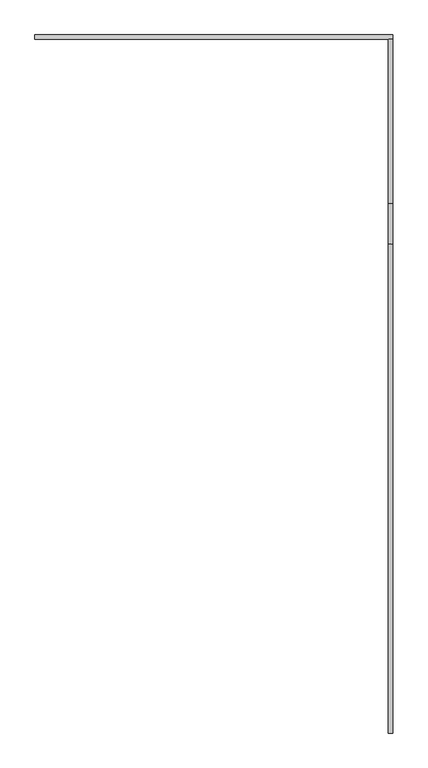
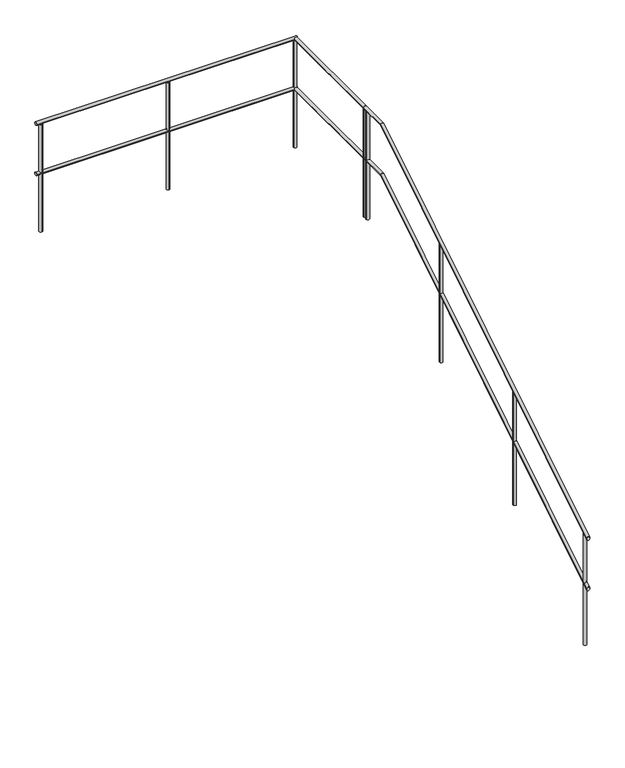
"""IFC4 building model written with IfcOpenShell, lengths in millimetres: railing geometry."""

from ifc_helpers import new_model, si_unit, point, frame, frame_2d, origin, place, context, project, spatial, circle_curve, ellipse_curve, trimmed, segment, composite_curve, outline, extrude, source, transform, mapped, element, save
from ifc_brep_helpers import plane_surface, cylinder_surface, advanced_brep


def railing_f57b0715(model_context):
    return source(origin(), model_context, "Body", "SolidModel", [
        advanced_brep(
        [(12685.1052251, 14699.5208589, 456.3396197), (12655.1052251, 14699.5208589, 456.3396197), (12685.1052251, 18339.5208589, 2547.0), (12655.1052251, 18339.5208589, 2547.0), (12685.1052251, 18063.8019306, 2547.0), (12655.1052251, 18063.8019306, 2547.0)],
        [
            (0, 1, ellipse_curve(frame((12670.1052251, 14699.5208589, 456.3396197), z_axis=(0.0, -1.0, 0.0), x_axis=(0.0, 0.0, -1.0)), 17.6603803, 15.0)),
            (1, 0, ellipse_curve(frame((12670.1052251, 14699.5208589, 456.3396197), z_axis=(0.0, -1.0, 0.0), x_axis=(0.0, 0.0, -1.0)), 17.6603803, 15.0)),
            (2, 3, circle_curve(frame((12670.1052251, 18339.5208589, 2547.0), z_axis=(0.0, 1.0, 0.0), x_axis=(-1.0, 0.0, 0.0)), 15.0)),
            (3, 2, circle_curve(frame((12670.1052251, 18339.5208589, 2547.0), z_axis=(0.0, 1.0, 0.0), x_axis=(-1.0, 0.0, 0.0)), 15.0)),
            (0, 4),
            (4, 5, ellipse_curve(frame((12670.1052251, 18063.8019306, 2547.0), z_axis=(0.0, -0.9616025257983003, -0.2744459552959912), x_axis=(0.0, 0.2744459552959914, -0.9616025257983002)), 15.5989607, 15.0)),
            (5, 1),
            (5, 4, ellipse_curve(frame((12670.1052251, 18063.8019306, 2547.0), z_axis=(0.0, -0.9616025257983003, -0.2744459552959912), x_axis=(0.0, 0.2744459552959914, -0.9616025257983002)), 15.5989607, 15.0)),
            (4, 2),
            (3, 5),
        ],
        [
            plane_surface(frame((12670.1052251, 14699.5208589, 474.0), z_axis=(0.0, -1.0, 0.0), x_axis=(0.0, 0.0, 1.0))),
            plane_surface(frame((12670.1052251, 18339.5208589, 2562.0), z_axis=(0.0, 1.0, 0.0), x_axis=(0.0, 0.0, 1.0))),
            cylinder_surface(frame((12670.1052251, 14707.4380966, 461.2596175), z_axis=(0.0, -0.8493588352433417, -0.5278158476155052), x_axis=(-1.0, 0.0, 0.0)), 15.0),
            cylinder_surface(frame((12670.1052251, 18059.5208589, 2547.0), z_axis=(0.0, -1.0, 0.0), x_axis=(-1.0, 0.0, 0.0)), 15.0),
        ],
        [
            (0, [[1, 2]]),
            (1, [[3, 4]]),
            (2, [[-1, 5, 6, 7]]),
            (2, [[-2, -7, 8, -5]]),
            (3, [[-6, 9, -4, 10]]),
            (3, [[-8, -10, -3, -9]]),
        ],
    ),
        advanced_brep(
        [(12685.1052251, 18339.5208589, 2547.0), (12655.1052251, 18339.5208589, 2547.0), (12685.1052251, 19469.5208589, 2547.0), (12655.1052251, 19469.5208589, 2547.0)],
        [
            (0, 1, circle_curve(frame((12670.1052251, 18339.5208589, 2547.0), z_axis=(0.0, -1.0, 0.0), x_axis=(-1.0, 0.0, 0.0)), 15.0)),
            (1, 0, circle_curve(frame((12670.1052251, 18339.5208589, 2547.0), z_axis=(0.0, -1.0, 0.0), x_axis=(-1.0, 0.0, 0.0)), 15.0)),
            (2, 3, circle_curve(frame((12670.1052251, 19469.5208589, 2547.0), z_axis=(0.0, 1.0, 0.0), x_axis=(-1.0, 0.0, 0.0)), 15.0)),
            (3, 2, circle_curve(frame((12670.1052251, 19469.5208589, 2547.0), z_axis=(0.0, 1.0, 0.0), x_axis=(-1.0, 0.0, 0.0)), 15.0)),
            (0, 2),
            (3, 1),
        ],
        [
            plane_surface(frame((12670.1052251, 18339.5208589, 2562.0), z_axis=(0.0, -1.0, 0.0), x_axis=(0.0, 0.0, 1.0))),
            plane_surface(frame((12670.1052251, 19469.5208589, 2562.0), z_axis=(0.0, 1.0, 0.0), x_axis=(0.0, 0.0, 1.0))),
            cylinder_surface(frame((12670.1052251, 18339.5208589, 2547.0), z_axis=(0.0, -1.0, 0.0), x_axis=(-1.0, 0.0, 0.0)), 15.0),
        ],
        [
            (0, [[1, 2]]),
            (1, [[3, 4]]),
            (2, [[-1, 5, -4, 6]]),
            (2, [[-2, -6, -3, -5]]),
        ],
    ),
        advanced_brep(
        [(12685.1052251, 19499.5208589, 2547.0), (12685.1052251, 19469.5208589, 2547.0), (10225.1052251, 19499.5208589, 2547.0), (10225.1052251, 19469.5208589, 2547.0)],
        [
            (0, 1, circle_curve(frame((12685.1052251, 19484.5208589, 2547.0), z_axis=(1.0, 0.0, 0.0), x_axis=(0.0, -1.0, 0.0)), 15.0)),
            (1, 0, circle_curve(frame((12685.1052251, 19484.5208589, 2547.0), z_axis=(1.0, 0.0, 0.0), x_axis=(0.0, -1.0, 0.0)), 15.0)),
            (2, 3, circle_curve(frame((10225.1052251, 19484.5208589, 2547.0), z_axis=(-1.0, 0.0, 0.0), x_axis=(0.0, -1.0, 0.0)), 15.0)),
            (3, 2, circle_curve(frame((10225.1052251, 19484.5208589, 2547.0), z_axis=(-1.0, 0.0, 0.0), x_axis=(0.0, -1.0, 0.0)), 15.0)),
            (0, 2),
            (3, 1),
        ],
        [
            plane_surface(frame((12685.1052251, 19484.5208589, 2562.0), z_axis=(1.0, 0.0, 0.0), x_axis=(0.0, -1.0, 0.0))),
            plane_surface(frame((10225.1052251, 19484.5208589, 2562.0), z_axis=(-1.0, 0.0, 0.0), x_axis=(0.0, -1.0, 0.0))),
            cylinder_surface(frame((12685.1052251, 19484.5208589, 2547.0), z_axis=(1.0, 0.0, 0.0), x_axis=(0.0, -1.0, 0.0)), 15.0),
        ],
        [
            (0, [[1, 2]]),
            (1, [[3, 4]]),
            (2, [[-1, 5, -4, 6]]),
            (2, [[-2, -6, -3, -5]]),
        ],
    ),
        advanced_brep(
        [(12685.1052251, 14699.5208589, 956.3396197), (12655.1052251, 14699.5208589, 956.3396197), (12685.1052251, 18063.8019306, 3047.0), (12655.1052251, 18063.8019306, 3047.0), (12685.1052251, 18339.5208589, 3047.0), (12655.1052251, 18339.5208589, 3047.0)],
        [
            (0, 1, ellipse_curve(frame((12670.1052251, 14699.5208589, 956.3396197), z_axis=(0.0, -1.0, 0.0), x_axis=(0.0, 0.0, -1.0)), 17.6603803, 15.0)),
            (1, 0, ellipse_curve(frame((12670.1052251, 14699.5208589, 956.3396197), z_axis=(0.0, -1.0, 0.0), x_axis=(0.0, 0.0, -1.0)), 17.6603803, 15.0)),
            (0, 2),
            (2, 3, ellipse_curve(frame((12670.1052251, 18063.8019306, 3047.0), z_axis=(0.0, -0.9616025257983003, -0.2744459552959912), x_axis=(0.0, 0.2744459552959914, -0.9616025257983002)), 15.5989607, 15.0)),
            (3, 1),
            (3, 2, ellipse_curve(frame((12670.1052251, 18063.8019306, 3047.0), z_axis=(0.0, -0.9616025257983003, -0.2744459552959912), x_axis=(0.0, 0.2744459552959914, -0.9616025257983002)), 15.5989607, 15.0)),
            (4, 5, circle_curve(frame((12670.1052251, 18339.5208589, 3047.0), z_axis=(0.0, 1.0, 0.0), x_axis=(-1.0, 0.0, 0.0)), 15.0)),
            (5, 4, circle_curve(frame((12670.1052251, 18339.5208589, 3047.0), z_axis=(0.0, 1.0, 0.0), x_axis=(-1.0, 0.0, 0.0)), 15.0)),
            (2, 4),
            (5, 3),
        ],
        [
            plane_surface(frame((12670.1052251, 14699.5208589, 974.0), z_axis=(0.0, -1.0, 0.0), x_axis=(0.0, 0.0, 1.0))),
            cylinder_surface(frame((12670.1052251, 14707.4380966, 961.2596175), z_axis=(0.0, -0.8493588352433417, -0.5278158476155052), x_axis=(-1.0, 0.0, 0.0)), 15.0),
            plane_surface(frame((12670.1052251, 18339.5208589, 3062.0), z_axis=(0.0, 1.0, 0.0), x_axis=(0.0, 0.0, 1.0))),
            cylinder_surface(frame((12670.1052251, 18059.5208589, 3047.0), z_axis=(0.0, -1.0, 0.0), x_axis=(-1.0, 0.0, 0.0)), 15.0),
        ],
        [
            (0, [[1, 2]]),
            (1, [[-1, 3, 4, 5]]),
            (1, [[-2, -5, 6, -3]]),
            (2, [[7, 8]]),
            (3, [[-4, 9, -8, 10]]),
            (3, [[-6, -10, -7, -9]]),
        ],
    ),
        advanced_brep(
        [(12685.1052251, 18339.5208589, 3047.0), (12655.1052251, 18339.5208589, 3047.0), (12685.1052251, 19469.5208589, 3047.0), (12655.1052251, 19469.5208589, 3047.0)],
        [
            (0, 1, circle_curve(frame((12670.1052251, 18339.5208589, 3047.0), z_axis=(0.0, -1.0, 0.0), x_axis=(-1.0, 0.0, 0.0)), 15.0)),
            (1, 0, circle_curve(frame((12670.1052251, 18339.5208589, 3047.0), z_axis=(0.0, -1.0, 0.0), x_axis=(-1.0, 0.0, 0.0)), 15.0)),
            (2, 3, circle_curve(frame((12670.1052251, 19469.5208589, 3047.0), z_axis=(0.0, 1.0, 0.0), x_axis=(-1.0, 0.0, 0.0)), 15.0)),
            (3, 2, circle_curve(frame((12670.1052251, 19469.5208589, 3047.0), z_axis=(0.0, 1.0, 0.0), x_axis=(-1.0, 0.0, 0.0)), 15.0)),
            (0, 2),
            (3, 1),
        ],
        [
            plane_surface(frame((12670.1052251, 18339.5208589, 3062.0), z_axis=(0.0, -1.0, 0.0), x_axis=(0.0, 0.0, 1.0))),
            plane_surface(frame((12670.1052251, 19469.5208589, 3062.0), z_axis=(0.0, 1.0, 0.0), x_axis=(0.0, 0.0, 1.0))),
            cylinder_surface(frame((12670.1052251, 18339.5208589, 3047.0), z_axis=(0.0, -1.0, 0.0), x_axis=(-1.0, 0.0, 0.0)), 15.0),
        ],
        [
            (0, [[1, 2]]),
            (1, [[3, 4]]),
            (2, [[-1, 5, -4, 6]]),
            (2, [[-2, -6, -3, -5]]),
        ],
    ),
        advanced_brep(
        [(12685.1052251, 19499.5208589, 3047.0), (12685.1052251, 19469.5208589, 3047.0), (10225.1052251, 19499.5208589, 3047.0), (10225.1052251, 19469.5208589, 3047.0)],
        [
            (0, 1, circle_curve(frame((12685.1052251, 19484.5208589, 3047.0), z_axis=(1.0, 0.0, 0.0), x_axis=(0.0, -1.0, 0.0)), 15.0)),
            (1, 0, circle_curve(frame((12685.1052251, 19484.5208589, 3047.0), z_axis=(1.0, 0.0, 0.0), x_axis=(0.0, -1.0, 0.0)), 15.0)),
            (2, 3, circle_curve(frame((10225.1052251, 19484.5208589, 3047.0), z_axis=(-1.0, 0.0, 0.0), x_axis=(0.0, -1.0, 0.0)), 15.0)),
            (3, 2, circle_curve(frame((10225.1052251, 19484.5208589, 3047.0), z_axis=(-1.0, 0.0, 0.0), x_axis=(0.0, -1.0, 0.0)), 15.0)),
            (0, 2),
            (3, 1),
        ],
        [
            plane_surface(frame((12685.1052251, 19484.5208589, 3062.0), z_axis=(1.0, 0.0, 0.0), x_axis=(0.0, -1.0, 0.0))),
            plane_surface(frame((10225.1052251, 19484.5208589, 3062.0), z_axis=(-1.0, 0.0, 0.0), x_axis=(0.0, -1.0, 0.0))),
            cylinder_surface(frame((12685.1052251, 19484.5208589, 3047.0), z_axis=(1.0, 0.0, 0.0), x_axis=(0.0, -1.0, 0.0)), 15.0),
        ],
        [
            (0, [[1, 2]]),
            (1, [[3, 4]]),
            (2, [[-1, 5, -4, 6]]),
            (2, [[-2, -6, -3, -5]]),
        ],
    ),
        extrude(outline(composite_curve([segment(trimmed(circle_curve(frame_2d((10270.1052251, 19484.5208589)), 15.0), [point((10270.1052251, 19469.5208589))], [point((10270.1052251, 19499.5208589))], False, "CARTESIAN"), True, "CONTINUOUS"), segment(trimmed(circle_curve(frame_2d((10270.1052251, 19484.5208589)), 15.0), [point((10270.1052251, 19499.5208589))], [point((10270.1052251, 19469.5208589))], False, "CARTESIAN"), True, "CONTINUOUS")], self_intersect=False)), frame((0.0, 0.0, 1962.0), z_axis=(0.0, 0.0, 1.0), x_axis=(1.0, 0.0, 0.0)), (0.0, 0.0, 1.0), 1070.0),
        extrude(outline(composite_curve([segment(trimmed(circle_curve(frame_2d((11470.1052251, 19484.5208589)), 15.0), [point((11470.1052251, 19469.5208589))], [point((11470.1052251, 19499.5208589))], False, "CARTESIAN"), True, "CONTINUOUS"), segment(trimmed(circle_curve(frame_2d((11470.1052251, 19484.5208589)), 15.0), [point((11470.1052251, 19499.5208589))], [point((11470.1052251, 19469.5208589))], False, "CARTESIAN"), True, "CONTINUOUS")], self_intersect=False)), frame((0.0, 0.0, 1962.0), z_axis=(0.0, 0.0, 1.0), x_axis=(1.0, 0.0, 0.0)), (0.0, 0.0, 1.0), 1070.0),
        extrude(outline(composite_curve([segment(trimmed(circle_curve(frame_2d((12670.1052251, 18299.5208589)), 15.0), [point((12655.1052251, 18299.5208589))], [point((12685.1052251, 18299.5208589))], False, "CARTESIAN"), True, "CONTINUOUS"), segment(trimmed(circle_curve(frame_2d((12670.1052251, 18299.5208589)), 15.0), [point((12685.1052251, 18299.5208589))], [point((12655.1052251, 18299.5208589))], False, "CARTESIAN"), True, "CONTINUOUS")], self_intersect=False)), frame((0.0, 0.0, 1962.0), z_axis=(0.0, 0.0, 1.0), x_axis=(1.0, 0.0, 0.0)), (0.0, 0.0, 1.0), 1070.0),
        extrude(outline(composite_curve([segment(trimmed(circle_curve(frame_2d((12670.1052251, 17099.5208589)), 15.0), [point((12655.1052251, 17099.5208589))], [point((12685.1052251, 17099.5208589))], False, "CARTESIAN"), True, "CONTINUOUS"), segment(trimmed(circle_curve(frame_2d((12670.1052251, 17099.5208589)), 15.0), [point((12685.1052251, 17099.5208589))], [point((12655.1052251, 17099.5208589))], False, "CARTESIAN"), True, "CONTINUOUS")], self_intersect=False)), frame((0.0, 0.0, 1266.0), z_axis=(0.0, 0.0, 1.0), x_axis=(1.0, 0.0, 0.0)), (0.0, 0.0, 1.0), 1169.4285714),
        extrude(outline(composite_curve([segment(trimmed(circle_curve(frame_2d((12670.1052251, 15899.5208589)), 15.0), [point((12655.1052251, 15899.5208589))], [point((12685.1052251, 15899.5208589))], False, "CARTESIAN"), True, "CONTINUOUS"), segment(trimmed(circle_curve(frame_2d((12670.1052251, 15899.5208589)), 15.0), [point((12685.1052251, 15899.5208589))], [point((12655.1052251, 15899.5208589))], False, "CARTESIAN"), True, "CONTINUOUS")], self_intersect=False)), frame((0.0, 0.0, 570.0), z_axis=(0.0, 0.0, 1.0), x_axis=(1.0, 0.0, 0.0)), (0.0, 0.0, 1.0), 1119.7142857),
        extrude(outline(composite_curve([segment(trimmed(circle_curve(frame_2d((12670.1052251, 19484.5208589)), 15.0), [point((12655.1052251, 19484.5208589))], [point((12685.1052251, 19484.5208589))], False, "CARTESIAN"), True, "CONTINUOUS"), segment(trimmed(circle_curve(frame_2d((12670.1052251, 19484.5208589)), 15.0), [point((12685.1052251, 19484.5208589))], [point((12655.1052251, 19484.5208589))], False, "CARTESIAN"), True, "CONTINUOUS")], self_intersect=False)), frame((0.0, 0.0, 1962.0), z_axis=(0.0, 0.0, 1.0), x_axis=(1.0, 0.0, 0.0)), (0.0, 0.0, 1.0), 1070.0),
        extrude(outline(composite_curve([segment(trimmed(circle_curve(frame_2d((12670.1052251, 18339.5208589)), 15.0), [point((12655.1052251, 18339.5208589))], [point((12685.1052251, 18339.5208589))], False, "CARTESIAN"), True, "CONTINUOUS"), segment(trimmed(circle_curve(frame_2d((12670.1052251, 18339.5208589)), 15.0), [point((12685.1052251, 18339.5208589))], [point((12655.1052251, 18339.5208589))], False, "CARTESIAN"), True, "CONTINUOUS")], self_intersect=False)), frame((0.0, 0.0, 1962.0), z_axis=(0.0, 0.0, 1.0), x_axis=(1.0, 0.0, 0.0)), (0.0, 0.0, 1.0), 1070.0),
        extrude(outline(composite_curve([segment(trimmed(circle_curve(frame_2d((10275.1052251, 19484.5208589)), 15.0), [point((10275.1052251, 19469.5208589))], [point((10275.1052251, 19499.5208589))], False, "CARTESIAN"), True, "CONTINUOUS"), segment(trimmed(circle_curve(frame_2d((10275.1052251, 19484.5208589)), 15.0), [point((10275.1052251, 19499.5208589))], [point((10275.1052251, 19469.5208589))], False, "CARTESIAN"), True, "CONTINUOUS")], self_intersect=False)), frame((0.0, 0.0, 1962.0), z_axis=(0.0, 0.0, 1.0), x_axis=(1.0, 0.0, 0.0)), (0.0, 0.0, 1.0), 1070.0),
        extrude(outline(composite_curve([segment(trimmed(circle_curve(frame_2d((12670.1052251, 14749.5208589)), 15.0), [point((12655.1052251, 14749.5208589))], [point((12685.1052251, 14749.5208589))], False, "CARTESIAN"), True, "CONTINUOUS"), segment(trimmed(circle_curve(frame_2d((12670.1052251, 14749.5208589)), 15.0), [point((12685.1052251, 14749.5208589))], [point((12655.1052251, 14749.5208589))], False, "CARTESIAN"), True, "CONTINUOUS")], self_intersect=False)), frame((0.0, 0.0, -126.0), z_axis=(0.0, 0.0, 1.0), x_axis=(1.0, 0.0, 0.0)), (0.0, 0.0, 1.0), 1101.0714286),
    ])


if __name__ == "__main__":
    model = new_model("IFC4")
    model_context = context("Model", 3, world=origin())
    ifc_project = project(units=[si_unit("LENGTHUNIT", "METRE", prefix="MILLI")], contexts=[model_context])
    site = spatial("IfcSite", under=ifc_project)
    building = spatial("IfcBuilding", under=site)
    placement = place(None, origin())
    railing_shape = railing_f57b0715(model_context)
    element("IfcRailing", 1, at=placement, inside=building, context=model_context, shape_type="MappedRepresentation", body=[
        mapped(railing_shape, transform((0.0, 0.0, 0.0), x_axis=(1.0, 0.0, 0.0), y_axis=(0.0, 1.0, 0.0), z_axis=(0.0, 0.0, 1.0))),
    ])
    save(model, "model.ifc")
